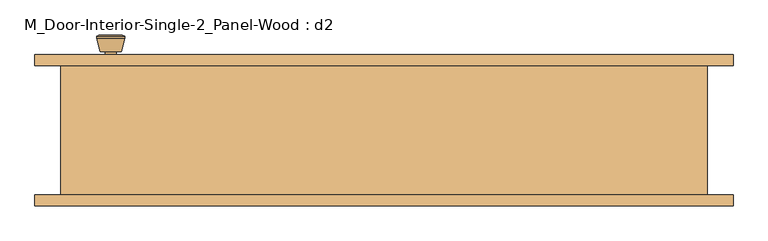
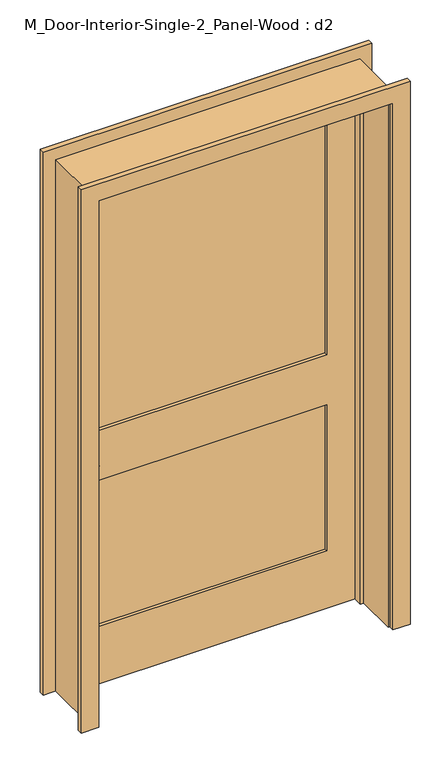
"""IFC4 building model written with IfcOpenShell, lengths in millimetres: door geometry, M_Door-Interior-Single-2_Panel-Wood : d2."""

from ifc_helpers import new_model, si_unit, point, frame, frame_2d, origin, place, context, project, spatial, polyline, circle_curve, trimmed, segment, composite_curve, outline, extrude, faceted_brep, source, transform, mapped, element, save
from ifc_brep_helpers import plane_surface, cylinder_surface, revolved_surface, advanced_brep


def m_door_interior_single_2_panel_wood_d2_be971991(model_context):
    return source(origin(), model_context, "Body", "SolidModel", [
        advanced_brep(
        [(-486.5, 70.825, 914.4), (-476.5, 70.825, 914.4), (-496.5, 70.825, 914.4), (-466.0241324, 21.825, 914.4), (-486.5, 21.825, 914.4), (-506.9758676, 21.825, 914.4), (-461.5, 23.6528681, 914.4), (-511.5, 23.6528681, 914.4), (-461.5, 27.1165463, 914.4), (-511.5, 27.1165463, 914.4), (-467.863764, 51.825, 914.4), (-505.136236, 51.825, 914.4), (-476.5, 51.825, 914.4), (-496.5, 51.825, 914.4)],
        [
            (0, 1),
            (1, 2, circle_curve(frame((-486.5, 70.825, 914.4), z_axis=(0.0, 1.0, 0.0), x_axis=(-1.0, 0.0, 0.0)), 10.0)),
            (2, 0),
            (2, 1, circle_curve(frame((-486.5, 70.825, 914.4), z_axis=(0.0, 1.0, 0.0), x_axis=(-1.0, 0.0, 0.0)), 10.0)),
            (3, 4),
            (4, 5),
            (5, 3, circle_curve(frame((-486.5, 21.825, 914.4), z_axis=(0.0, -1.0, 0.0), x_axis=(-1.0, 0.0, 0.0)), 20.4758676)),
            (3, 5, circle_curve(frame((-486.5, 21.825, 914.4), z_axis=(0.0, -1.0, 0.0), x_axis=(-1.0, 0.0, 0.0)), 20.4758676)),
            (6, 3),
            (5, 7),
            (7, 6, circle_curve(frame((-486.5, 23.6528681, 914.4), z_axis=(0.0, -1.0, 0.0), x_axis=(-1.0, 0.0, 0.0)), 25.0)),
            (6, 7, circle_curve(frame((-486.5, 23.6528681, 914.4), z_axis=(0.0, -1.0, 0.0), x_axis=(-1.0, 0.0, 0.0)), 25.0)),
            (8, 6),
            (7, 9),
            (9, 8, circle_curve(frame((-486.5, 27.1165463, 914.4), z_axis=(0.0, -1.0, 0.0), x_axis=(-1.0, 0.0, 0.0)), 25.0)),
            (8, 9, circle_curve(frame((-486.5, 27.1165463, 914.4), z_axis=(0.0, -1.0, 0.0), x_axis=(-1.0, 0.0, 0.0)), 25.0)),
            (10, 8),
            (9, 11),
            (11, 10, circle_curve(frame((-486.5, 51.825, 914.4), z_axis=(0.0, -1.0, 0.0), x_axis=(-1.0, 0.0, 0.0)), 18.636236)),
            (10, 11, circle_curve(frame((-486.5, 51.825, 914.4), z_axis=(0.0, -1.0, 0.0), x_axis=(-1.0, 0.0, 0.0)), 18.636236)),
            (12, 10),
            (11, 13),
            (13, 12, circle_curve(frame((-486.5, 51.825, 914.4), z_axis=(0.0, -1.0, 0.0), x_axis=(-1.0, 0.0, 0.0)), 10.0)),
            (12, 13, circle_curve(frame((-486.5, 51.825, 914.4), z_axis=(0.0, -1.0, 0.0), x_axis=(-1.0, 0.0, 0.0)), 10.0)),
            (1, 12),
            (13, 2),
        ],
        [
            plane_surface(frame((-486.5, 70.825, 914.4), z_axis=(0.0, 1.0, 0.0), x_axis=(-1.0, 0.0, 0.0))),
            plane_surface(frame((-486.5, 21.825, 914.4), z_axis=(0.0, -1.0, 0.0), x_axis=(-1.0, 0.0, 0.0))),
            revolved_surface(polyline([(-506.9758676, 21.825, 914.4), (-511.5, 23.6528681, 914.4)]), (-486.5, 70.825, 914.4), (0.0, 1.0, 0.0)),
            cylinder_surface(frame((-486.5, 70.825, 914.4), z_axis=(0.0, 1.0, 0.0), x_axis=(-1.0, 0.0, 0.0)), 25.0),
            revolved_surface(polyline([(-511.5, 27.1165463, 914.4), (-505.136236, 51.825, 914.4)]), (-486.5, 70.825, 914.4), (0.0, 1.0, 0.0)),
            plane_surface(frame((-486.5, 51.825, 914.4), z_axis=(0.0, 1.0, 0.0), x_axis=(-1.0, 0.0, 0.0))),
            cylinder_surface(frame((-486.5, 70.825, 914.4), z_axis=(0.0, 1.0, 0.0), x_axis=(-1.0, 0.0, 0.0)), 10.0),
        ],
        [
            (0, [[1, 2, 3]]),
            (0, [[-3, 4, -1]]),
            (1, [[5, 6, 7]]),
            (1, [[-6, -5, 8]]),
            (2, [[9, -7, 10, 11]]),
            (2, [[-10, -8, -9, 12]]),
            (3, [[13, -11, 14, 15]]),
            (3, [[-14, -12, -13, 16]]),
            (4, [[17, -15, 18, 19]]),
            (4, [[-18, -16, -17, 20]]),
            (5, [[21, -19, 22, 23]]),
            (5, [[-22, -20, -21, 24]]),
            (6, [[25, -23, 26, -2]]),
            (6, [[-26, -24, -25, -4]]),
        ],
    ),
        extrude(outline(composite_curve([segment(trimmed(circle_curve(frame_2d((914.4, -486.5)), 30.0), [point((914.4, -516.5))], [point((914.4, -456.5))], False, "CARTESIAN"), True, "CONTINUOUS"), segment(trimmed(circle_curve(frame_2d((914.4, -486.5)), 30.0), [point((914.4, -456.5))], [point((914.4, -516.5))], False, "CARTESIAN"), True, "CONTINUOUS")], self_intersect=False)), frame((0.0, 70.825, 0.0), z_axis=(0.0, 1.0, 0.0), x_axis=(0.0, 0.0, 1.0)), (0.0, 0.0, 1.0), 6.0),
        advanced_brep(
        [(-486.5, 117.825, 914.4), (-496.5, 117.825, 914.4), (-476.5, 117.825, 914.4), (-466.0241324, 166.825, 914.4), (-506.9758676, 166.825, 914.4), (-486.5, 166.825, 914.4), (-461.5, 164.9971319, 914.4), (-511.5, 164.9971319, 914.4), (-461.5, 161.5334537, 914.4), (-511.5, 161.5334537, 914.4), (-467.863764, 136.825, 914.4), (-505.136236, 136.825, 914.4), (-476.5, 136.825, 914.4), (-496.5, 136.825, 914.4)],
        [
            (0, 1),
            (1, 2, circle_curve(frame((-486.5, 117.825, 914.4), z_axis=(0.0, -1.0, 0.0), x_axis=(-1.0, 0.0, 0.0)), 10.0)),
            (2, 0),
            (2, 1, circle_curve(frame((-486.5, 117.825, 914.4), z_axis=(0.0, -1.0, 0.0), x_axis=(-1.0, 0.0, 0.0)), 10.0)),
            (3, 4, circle_curve(frame((-486.5, 166.825, 914.4), z_axis=(0.0, 1.0, 0.0), x_axis=(-1.0, 0.0, 0.0)), 20.4758676)),
            (4, 5),
            (5, 3),
            (4, 3, circle_curve(frame((-486.5, 166.825, 914.4), z_axis=(0.0, 1.0, 0.0), x_axis=(-1.0, 0.0, 0.0)), 20.4758676)),
            (6, 7, circle_curve(frame((-486.5, 164.9971319, 914.4), z_axis=(0.0, 1.0, 0.0), x_axis=(-1.0, 0.0, 0.0)), 25.0)),
            (7, 4),
            (3, 6),
            (7, 6, circle_curve(frame((-486.5, 164.9971319, 914.4), z_axis=(0.0, 1.0, 0.0), x_axis=(-1.0, 0.0, 0.0)), 25.0)),
            (8, 9, circle_curve(frame((-486.5, 161.5334537, 914.4), z_axis=(0.0, 1.0, 0.0), x_axis=(-1.0, 0.0, 0.0)), 25.0)),
            (9, 7),
            (6, 8),
            (9, 8, circle_curve(frame((-486.5, 161.5334537, 914.4), z_axis=(0.0, 1.0, 0.0), x_axis=(-1.0, 0.0, 0.0)), 25.0)),
            (10, 11, circle_curve(frame((-486.5, 136.825, 914.4), z_axis=(0.0, 1.0, 0.0), x_axis=(-1.0, 0.0, 0.0)), 18.636236)),
            (11, 9),
            (8, 10),
            (11, 10, circle_curve(frame((-486.5, 136.825, 914.4), z_axis=(0.0, 1.0, 0.0), x_axis=(-1.0, 0.0, 0.0)), 18.636236)),
            (12, 13, circle_curve(frame((-486.5, 136.825, 914.4), z_axis=(0.0, 1.0, 0.0), x_axis=(-1.0, 0.0, 0.0)), 10.0)),
            (13, 11),
            (10, 12),
            (13, 12, circle_curve(frame((-486.5, 136.825, 914.4), z_axis=(0.0, 1.0, 0.0), x_axis=(-1.0, 0.0, 0.0)), 10.0)),
            (1, 13),
            (12, 2),
        ],
        [
            plane_surface(frame((-486.5, 117.825, 914.4), z_axis=(0.0, -1.0, 0.0), x_axis=(-1.0, 0.0, 0.0))),
            plane_surface(frame((-486.5, 166.825, 914.4), z_axis=(0.0, 1.0, 0.0), x_axis=(-1.0, 0.0, 0.0))),
            revolved_surface(polyline([(-506.9758676, 166.825, 914.4), (-511.5, 164.9971319, 914.4)]), (-486.5, 117.825, 914.4), (0.0, -1.0, 0.0)),
            cylinder_surface(frame((-486.5, 117.825, 914.4), z_axis=(0.0, -1.0, 0.0), x_axis=(-1.0, 0.0, 0.0)), 25.0),
            revolved_surface(polyline([(-511.5, 161.5334537, 914.4), (-505.136236, 136.825, 914.4)]), (-486.5, 117.825, 914.4), (0.0, -1.0, 0.0)),
            plane_surface(frame((-486.5, 136.825, 914.4), z_axis=(0.0, -1.0, 0.0), x_axis=(-1.0, 0.0, 0.0))),
            cylinder_surface(frame((-486.5, 117.825, 914.4), z_axis=(0.0, -1.0, 0.0), x_axis=(-1.0, 0.0, 0.0)), 10.0),
        ],
        [
            (0, [[1, 2, 3]]),
            (0, [[-3, 4, -1]]),
            (1, [[5, 6, 7]]),
            (1, [[8, -7, -6]]),
            (2, [[9, 10, -5, 11]]),
            (2, [[12, -11, -8, -10]]),
            (3, [[13, 14, -9, 15]]),
            (3, [[16, -15, -12, -14]]),
            (4, [[17, 18, -13, 19]]),
            (4, [[20, -19, -16, -18]]),
            (5, [[21, 22, -17, 23]]),
            (5, [[24, -23, -20, -22]]),
            (6, [[-2, 25, -21, 26]]),
            (6, [[-4, -26, -24, -25]]),
        ],
    ),
        extrude(outline(composite_curve([segment(trimmed(circle_curve(frame_2d((914.4, -486.5)), 30.0), [point((914.4, -516.5))], [point((914.4, -456.5))], False, "CARTESIAN"), True, "CONTINUOUS"), segment(trimmed(circle_curve(frame_2d((914.4, -486.5)), 30.0), [point((914.4, -456.5))], [point((914.4, -516.5))], False, "CARTESIAN"), True, "CONTINUOUS")], self_intersect=False)), frame((0.0, 111.825, 0.0), z_axis=(0.0, 1.0, 0.0), x_axis=(0.0, 0.0, 1.0)), (0.0, 0.0, 1.0), 6.0),
        extrude(outline(polyline([(430.0, 88.4916667), (-430.0, 88.4916667), (-430.0, 100.1583333), (430.0, 100.1583333), (430.0, 88.4916667)])), frame((0.0, 0.0, 1014.4), z_axis=(0.0, 0.0, 1.0), x_axis=(1.0, 0.0, 0.0)), (0.0, 0.0, 1.0), 965.6),
        extrude(outline(polyline([(430.0, 88.4916667), (-430.0, 88.4916667), (-430.0, 100.1583333), (430.0, 100.1583333), (430.0, 88.4916667)])), frame((0.0, 0.0, 230.0), z_axis=(0.0, 0.0, 1.0), x_axis=(1.0, 0.0, 0.0)), (0.0, 0.0, 1.0), 584.4),
        extrude(outline(polyline([(2100.0, -550.0), (0.0, -550.0), (0.0, 550.0), (2100.0, 550.0), (2100.0, -550.0)]), holes=[polyline([(1980.0, -430.0), (1980.0, 430.0), (1014.4, 430.0), (1014.4, -430.0), (1980.0, -430.0)]), polyline([(814.4, -430.0), (814.4, 430.0), (230.0, 430.0), (230.0, -430.0), (814.4, -430.0)])]), frame((0.0, 76.825, 0.0), z_axis=(0.0, 1.0, 0.0), x_axis=(0.0, 0.0, 1.0)), (0.0, 0.0, 1.0), 35.0),
        faceted_brep([(575.0, 111.825, 0.0), (575.0, -118.175, 0.0), (550.0, -118.175, 0.0), (550.0, 41.9, 0.0), (537.3, 41.9, 0.0), (537.3, 76.825, 0.0), (550.0, 76.825, 0.0), (550.0, 111.825, 0.0), (575.0, 111.825, 2125.0), (575.0, -118.175, 2125.0), (-575.0, -118.175, 2125.0), (-575.0, -118.175, 0.0), (-550.0, -118.175, 0.0), (-550.0, -118.175, 2100.0), (550.0, -118.175, 2100.0), (550.0, 41.9, 2100.0), (-550.0, 41.9, 2100.0), (-550.0, 41.9, 0.0), (-537.3, 41.9, 0.0), (-537.3, 41.9, 2087.3), (537.3, 41.9, 2087.3), (537.3, 76.825, 2087.3), (-537.3, 76.825, 2087.3), (-537.3, 76.825, 0.0), (-550.0, 76.825, 0.0), (-550.0, 76.825, 2100.0), (550.0, 76.825, 2100.0), (550.0, 111.825, 2100.0), (-550.0, 111.825, 2100.0), (-550.0, 111.825, 0.0), (-575.0, 111.825, 0.0), (-575.0, 111.825, 2125.0)], [[[0, 1, 2, 3, 4, 5, 6, 7]], [[1, 0, 8, 9]], [[2, 1, 9, 10, 11, 12, 13, 14]], [[3, 2, 14, 15]], [[4, 3, 15, 16, 17, 18, 19, 20]], [[5, 4, 20, 21]], [[6, 5, 21, 22, 23, 24, 25, 26]], [[7, 6, 26, 27]], [[0, 7, 27, 28, 29, 30, 31, 8]], [[9, 8, 31, 10]], [[15, 14, 13, 16]], [[21, 20, 19, 22]], [[27, 26, 25, 28]], [[30, 29, 24, 23, 18, 17, 12, 11]], [[10, 31, 30, 11]], [[16, 13, 12, 17]], [[22, 19, 18, 23]], [[28, 25, 24, 29]]]),
        extrude(outline(polyline([(0.0, 556.35), (0.0, 621.35), (2171.35, 621.35), (2171.35, -621.35), (0.0, -621.35), (0.0, -556.35), (2106.35, -556.35), (2106.35, 556.35), (0.0, 556.35)])), frame((0.0, -138.175, 0.0), z_axis=(0.0, 1.0, 0.0), x_axis=(0.0, 0.0, 1.0)), (0.0, 0.0, 1.0), 20.0),
        extrude(outline(polyline([(0.0, 556.35), (0.0, 621.35), (2171.35, 621.35), (2171.35, -621.35), (0.0, -621.35), (0.0, -556.35), (2106.35, -556.35), (2106.35, 556.35), (0.0, 556.35)])), frame((0.0, 111.825, 0.0), z_axis=(0.0, 1.0, 0.0), x_axis=(0.0, 0.0, 1.0)), (0.0, 0.0, 1.0), 20.0),
    ])


if __name__ == "__main__":
    model = new_model("IFC4")
    model_context = context("Model", 3, world=origin())
    ifc_project = project(units=[si_unit("LENGTHUNIT", "METRE", prefix="MILLI")], contexts=[model_context])
    site = spatial("IfcSite", under=ifc_project)
    building = spatial("IfcBuilding", under=site)
    placement = place(None, origin())
    m_door_interior_single_2_panel_wood_d2_shape = m_door_interior_single_2_panel_wood_d2_be971991(model_context)
    element("IfcDoor", 1, ObjectType="M_Door-Interior-Single-2_Panel-Wood : d2", at=placement, inside=building, context=model_context, shape_type="MappedRepresentation", body=[
        mapped(m_door_interior_single_2_panel_wood_d2_shape, transform((0.0, 0.0, 0.0), x_axis=(1.0, 0.0, 0.0), y_axis=(0.0, 1.0, 0.0), z_axis=(0.0, 0.0, 1.0))),
    ])
    save(model, "model.ifc")

# Revit data of these elements
# Type "M_Door-Interior-Single-2_Panel-Wood : d2"
#   Type Mark = "53"
#   Assembly Code = "C1020300"
#   Analytic Construction = "Wooden"
#   Top Rail = 12 cm
#   Thickness = 3.5 cm
#   Thermal Resistance (R) = 0.455703 (m²·K)/W
#   Swing Angle [instance default] = 90.00°
#   Stiles = 12 cm
#   Rough Width = 115 cm
#   Rough Height = 212.5 cm
#   Lock Rail = 20 cm
#   Height = 210 cm
#   Width = 110 cm
#   Heat Transfer Coefficient (U) = 2.19465 W/(m²·K)
#   Bottom Rail = 23 cm
#   Trim Material = Cherry
#   Panel Material = Cherry
#   Frame Material = Cherry
#   Door Handle Material = Aluminum
#   Visual Light Transmittance = 0
#   Solar Heat Gain Coefficient = 0
#   Wall Closure = (empty or 0)
#   Function = (empty or 0)
# Element 1 (IfcDoor, "M_Door-Interior-Single-2_Panel-Wood : d2")
#   Materials on its faces: "Cherry", "Aluminum"
# Materials
#   "Cherry": class "Wood", colour RGB 226 177 128, transparency 0, Description = "Prunus Serotina", Cost = 0
#   "Aluminum": class "Metal", colour RGB 247 247 247, transparency 0, Description = "Aluminum 6061", Cost = 0
